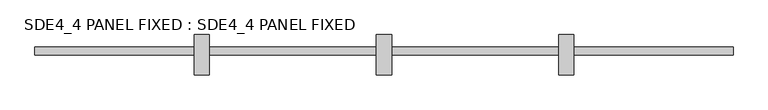
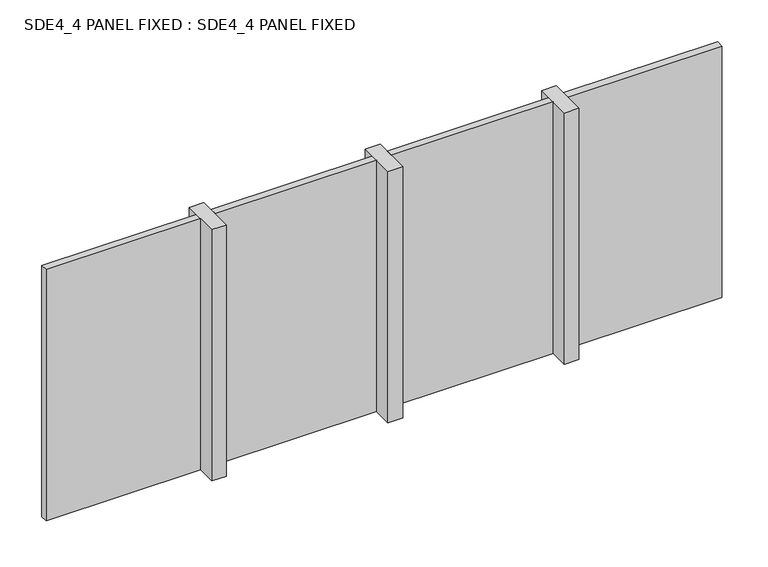
"""IFC4 building model written with IfcOpenShell, lengths in millimetres: plate geometry, SDE4_4 PANEL FIXED : SDE4_4 PANEL FIXED."""

from ifc_helpers import new_model, si_unit, origin, origin_with_axes, place, context, project, spatial, polyline, outline, extrude, source, transform, mapped, element, save


def sde4_4_panel_fixed_sde4_4_panel_fixed_ee0e71f4(model_context):
    return source(origin(), model_context, "Body", "SweptSolid", [
        extrude(outline(polyline([(-1150.0, 132.5), (-1150.0, -132.5), (-1250.0, -132.5), (-1250.0, 132.5), (-1150.0, 132.5)])), origin_with_axes(), (0.0, 0.0, 1.0), 1810.0),
        extrude(outline(polyline([(50.0, 132.5), (50.0, -132.5), (-50.0, -132.5), (-50.0, 132.5), (50.0, 132.5)])), origin_with_axes(), (0.0, 0.0, 1.0), 1810.0),
        extrude(outline(polyline([(1250.0, 132.5), (1250.0, -132.5), (1150.0, -132.5), (1150.0, 132.5), (1250.0, 132.5)])), origin_with_axes(), (0.0, 0.0, 1.0), 1810.0),
        extrude(outline(polyline([(2299.0, 50.0), (2299.0, 0.0), (1250.0, 0.0), (1250.0, 50.0), (2299.0, 50.0)])), origin_with_axes(), (0.0, 0.0, 1.0), 1810.0),
        extrude(outline(polyline([(1150.0, 50.0), (1150.0, 0.0), (50.0, 0.0), (50.0, 50.0), (1150.0, 50.0)])), origin_with_axes(), (0.0, 0.0, 1.0), 1810.0),
        extrude(outline(polyline([(-50.0, 50.0), (-50.0, 0.0), (-1150.0, 0.0), (-1150.0, 50.0), (-50.0, 50.0)])), origin_with_axes(), (0.0, 0.0, 1.0), 1810.0),
        extrude(outline(polyline([(-1250.0, 50.0), (-1250.0, 0.0), (-2300.0, 0.0), (-2300.0, 50.0), (-1250.0, 50.0)])), origin_with_axes(), (0.0, 0.0, 1.0), 1810.0),
    ])


if __name__ == "__main__":
    model = new_model("IFC4")
    model_context = context("Model", 3, world=origin())
    ifc_project = project(units=[si_unit("LENGTHUNIT", "METRE", prefix="MILLI")], contexts=[model_context])
    site = spatial("IfcSite", under=ifc_project)
    building = spatial("IfcBuilding", under=site)
    placement = place(None, origin())
    sde4_4_panel_fixed_sde4_4_panel_fixed_shape = sde4_4_panel_fixed_sde4_4_panel_fixed_ee0e71f4(model_context)
    element("IfcPlate", 1, ObjectType="SDE4_4 PANEL FIXED : SDE4_4 PANEL FIXED", at=placement, inside=building, context=model_context, shape_type="MappedRepresentation", body=[
        mapped(sde4_4_panel_fixed_sde4_4_panel_fixed_shape, transform((0.0, 0.0, 0.0), x_axis=(1.0, 0.0, 0.0), y_axis=(0.0, 1.0, 0.0), z_axis=(0.0, 0.0, 1.0))),
    ])
    save(model, "model.ifc")

# Revit data of these elements
# Type "SDE4_4 PANEL FIXED : SDE4_4 PANEL FIXED"
#   Type Mark = "CW-GLASS"
#   Analytic Construction = "<None>"
#   Glass = Glass
#   Frame = Aluminium
# Element 1 (IfcPlate, "SDE4_4 PANEL FIXED : SDE4_4 PANEL FIXED")
#   Materials on its faces: "Glass", "Aluminium"
# Materials
#   "Glass": class "Glass", colour RGB 0 128 192, transparency 0.9, Keynote = "L40", Cost = 0
#   "Aluminium": class "Unassigned", colour RGB 247 247 247, transparency 0, Cost = 0
